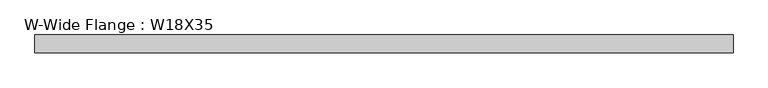
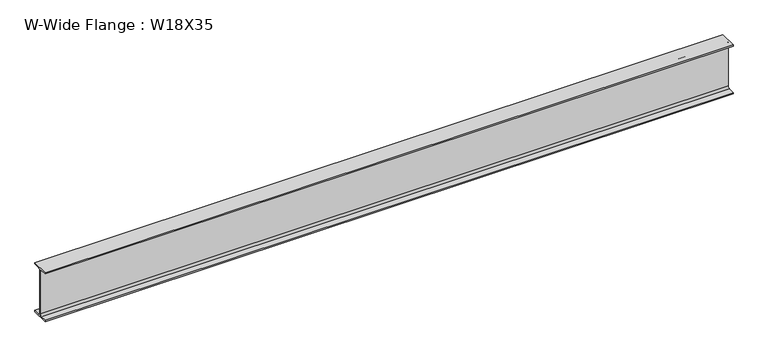
"""IFC4 building model written with IfcOpenShell, lengths in millimetres: beam geometry, W-Wide Flange : W18X35."""

from ifc_helpers import new_model, si_unit, point, frame, frame_2d, origin, place, context, project, spatial, polyline, circle_curve, trimmed, segment, composite_curve, outline, extrude, source, transform, mapped, element, save


def w_wide_flange_w18x35_6a08477e(model_context):
    return source(origin(), model_context, "Body", "SweptSolid", [
        extrude(outline(composite_curve([segment(polyline([(76.2, -213.995), (76.2, -224.79), (-76.2, -224.79), (-76.2, -213.995), (-21.59, -213.995)]), True, "CONTINUOUS"), segment(trimmed(circle_curve(frame_2d((-21.59, -196.215)), 17.78), [point((-21.59, -213.995))], [point((-3.81, -196.215))], True, "CARTESIAN"), True, "CONTINUOUS"), segment(polyline([(-3.81, -196.215), (-3.81, 196.215)]), True, "CONTINUOUS"), segment(trimmed(circle_curve(frame_2d((-21.59, 196.215)), 17.78), [point((-3.81, 196.215))], [point((-21.59, 213.995))], True, "CARTESIAN"), True, "CONTINUOUS"), segment(polyline([(-21.59, 213.995), (-76.2, 213.995), (-76.2, 224.79), (76.2, 224.79), (76.2, 213.995), (21.59, 213.995)]), True, "CONTINUOUS"), segment(trimmed(circle_curve(frame_2d((21.59, 196.215)), 17.78), [point((21.59, 213.995))], [point((3.81, 196.215))], True, "CARTESIAN"), True, "CONTINUOUS"), segment(polyline([(3.81, 196.215), (3.81, -196.215)]), True, "CONTINUOUS"), segment(trimmed(circle_curve(frame_2d((21.59, -196.215)), 17.78), [point((3.81, -196.215))], [point((21.59, -213.995))], True, "CARTESIAN"), True, "CONTINUOUS"), segment(polyline([(21.59, -213.995), (76.2, -213.995)]), True, "CONTINUOUS")], self_intersect=False)), frame((-2997.2, 0.0, 0.0), z_axis=(1.0, 0.0, 0.0), x_axis=(0.0, 1.0, 0.0)), (0.0, 0.0, 1.0), 5994.4),
    ])


if __name__ == "__main__":
    model = new_model("IFC4")
    model_context = context("Model", 3, world=origin())
    ifc_project = project(units=[si_unit("LENGTHUNIT", "METRE", prefix="MILLI")], contexts=[model_context])
    site = spatial("IfcSite", under=ifc_project)
    building = spatial("IfcBuilding", under=site)
    placement = place(None, origin())
    w_wide_flange_w18x35_shape = w_wide_flange_w18x35_6a08477e(model_context)
    element("IfcBeam", 1, ObjectType="W-Wide Flange : W18X35", at=placement, inside=building, context=model_context, shape_type="MappedRepresentation", body=[
        mapped(w_wide_flange_w18x35_shape, transform((0.0, 0.0, 0.0), x_axis=(1.0, 0.0, 0.0), y_axis=(0.0, 1.0, 0.0), z_axis=(0.0, 0.0, 1.0))),
    ])
    save(model, "model.ifc")

# Revit data of these elements
# Type "W-Wide Flange : W18X35"
#   Assembly Code = "B10"
#   W = 35
#   Length [instance default] = 5' - 0"
#   bf = 0' - 6"
#   d = 1' - 5.7"
#   k = 0' - 1 1/8"
#   k2 = 0' - 0.7"
#   tf = 0' - 0.425"
#   tw = 0' - 0.3"
#   A = 0.0715278 SF
#   Structural Material [instance default] = Steel ASTM A992
# Element 1 (IfcBeam, "W-Wide Flange : W18X35")
#   Materials on its faces: "Steel ASTM A992"
# Materials
#   "Steel ASTM A992": class "Metal", colour RGB 199 199 199, transparency 0, Description = "Structural steel 50ksi", Cost = 0
